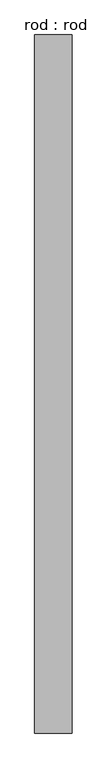
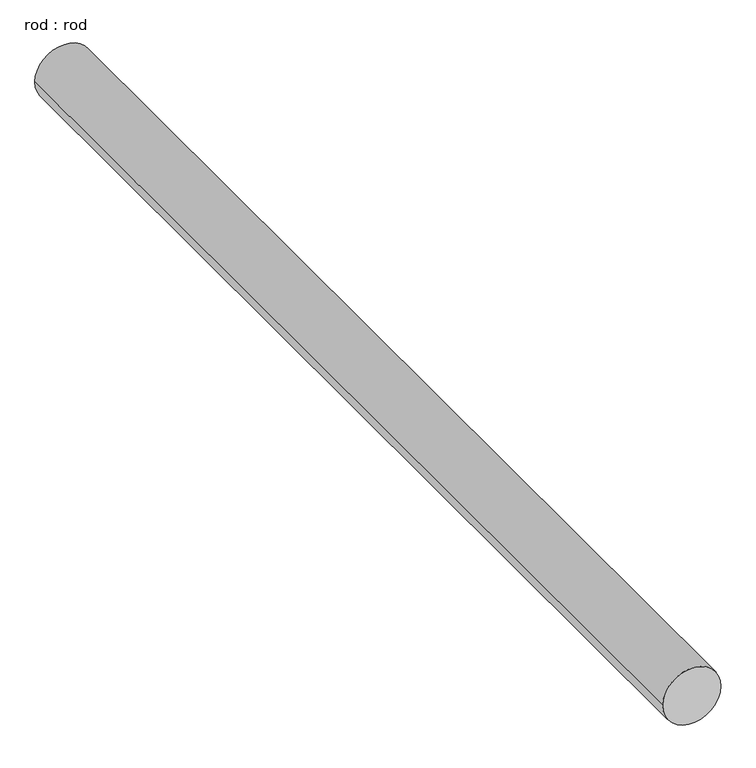
"""IFC4 building model written with IfcOpenShell, lengths in millimetres: proxy geometry, rod : rod."""

import ifcopenshell
import ifcopenshell.guid

model = None  # the IFC model being written
_history = None  # IfcOwnerHistory: only IFC2X3 demands one
_inside = {}  # id of a spatial element -> (the spatial element, [elements in it])
_under = {}  # id of a project, library or spatial element -> (it, [spatial elements below it])
_declared = {}  # id of a project -> (the project, [libraries it declares])
_typed = {}  # id of a type object -> (the type object, [elements of that type])
_made_of = {}  # id of a material, layer set ... -> (it, [elements and type objects made of it])


def new_model(schema):
    """Start an empty IFC model of exactly this schema.

    Asked for "IFC4X3", IfcOpenShell would pick the latest addendum, in which some entities
    have other attributes; the version numbers below select the first issue.
    IFC2X3 requires an IfcOwnerHistory on every rooted entity: one is made here for all.
    """
    global model, _history
    if schema == "IFC4X3":
        model = ifcopenshell.file(schema_version=(4, 3, 0, 0))
    else:
        model = ifcopenshell.file(schema=schema)
    _inside.clear()
    _under.clear()
    _declared.clear()
    _typed.clear()
    _made_of.clear()
    _history = None
    if model.schema == "IFC2X3":
        org = make("IfcOrganization", Name="unknown")
        user = make(
            "IfcPersonAndOrganization",
            ThePerson=make("IfcPerson", FamilyName="unknown"),
            TheOrganization=org,
        )
        app = make(
            "IfcApplication",
            ApplicationDeveloper=org,
            Version="unknown",
            ApplicationFullName="unknown",
            ApplicationIdentifier="unknown",
        )
        _history = make(
            "IfcOwnerHistory",
            OwningUser=user,
            OwningApplication=app,
            ChangeAction="ADDED",
            CreationDate=0,
        )
    return model


def make(cls, **values):
    """One entity of the class cls with the attributes given. An attribute that is None is left unset."""
    return model.create_entity(
        cls, **{name: value for name, value in values.items() if value is not None}
    )


def rooted(cls, **values):
    """An entity with a GlobalId (a new one), such as an element, a storey or a relation."""
    return make(cls, GlobalId=ifcopenshell.guid.new(), OwnerHistory=_history, **values)


def si_unit(unit_type, name, prefix=None):
    """IfcSIUnit, for example si_unit("LENGTHUNIT", "METRE", prefix="MILLI")."""
    return make("IfcSIUnit", UnitType=unit_type, Prefix=prefix, Name=name)


def assignment(units):
    """IfcUnitAssignment: the units of a project."""
    return None if units is None else make("IfcUnitAssignment", Units=units)


def point(xyz):
    """IfcCartesianPoint."""
    return None if xyz is None else make("IfcCartesianPoint", Coordinates=xyz)


def direction(xyz):
    """IfcDirection."""
    return None if xyz is None else make("IfcDirection", DirectionRatios=xyz)


def frame(location, z_axis=None, x_axis=None):
    """IfcAxis2Placement3D, a coordinate frame: its origin and axes. An axis left out is left unset."""
    return make(
        "IfcAxis2Placement3D",
        Location=point(location),
        Axis=direction(z_axis),
        RefDirection=direction(x_axis),
    )


def frame_2d(location, x_axis=None):
    """IfcAxis2Placement2D, a coordinate frame in the plane: its origin and x axis."""
    return make(
        "IfcAxis2Placement2D", Location=point(location), RefDirection=direction(x_axis)
    )


def origin():
    """The frame at (0, 0, 0) with its axes left unset."""
    return frame((0.0, 0.0, 0.0))


def place(relative_to, where):
    """IfcLocalPlacement: puts the frame where relative to a parent placement (None: the world)."""
    return make(
        "IfcLocalPlacement", PlacementRelTo=relative_to, RelativePlacement=where
    )


def context(
    kind, dimensions, precision=None, world=None, true_north=None, identifier=None
):
    """IfcGeometricRepresentationContext, for example the 3D "Model" context."""
    return make(
        "IfcGeometricRepresentationContext",
        ContextIdentifier=identifier,
        ContextType=kind,
        CoordinateSpaceDimension=dimensions,
        Precision=precision,
        WorldCoordinateSystem=world,
        TrueNorth=true_north,
    )


def project(units=None, contexts=None):
    """IfcProject with its units and contexts."""
    return rooted(
        "IfcProject",
        Name="project",
        RepresentationContexts=contexts,
        UnitsInContext=assignment(units),
    )


def spatial(cls, under=None, at=None, **own):
    """A site, building, storey or space (cls), placed at a placement, below another one or the project."""
    s = rooted(cls, ObjectPlacement=at, **own)
    if under is not None:
        _under.setdefault(under.id(), (under, []))[1].append(s)
    return s


def circle_curve(where, radius):
    """IfcCircle in the frame where."""
    return make("IfcCircle", Position=where, Radius=radius)


def trimmed(basis, trim1, trim2, sense, master):
    """IfcTrimmedCurve: the piece of a basis curve between two trims."""
    return make(
        "IfcTrimmedCurve",
        BasisCurve=basis,
        Trim1=trim1,
        Trim2=trim2,
        SenseAgreement=sense,
        MasterRepresentation=master,
    )


def segment(curve, same_sense, transition):
    """IfcCompositeCurveSegment."""
    return make(
        "IfcCompositeCurveSegment",
        Transition=transition,
        SameSense=same_sense,
        ParentCurve=curve,
    )


def composite_curve(segments, self_intersect=None):
    """IfcCompositeCurve: segments joined end to end."""
    return make("IfcCompositeCurve", Segments=segments, SelfIntersect=self_intersect)


def outline(outer, holes=None, kind="AREA"):
    """IfcArbitraryClosedProfileDef: a profile drawn as a closed curve; with holes, ...WithVoids."""
    if holes is None:
        return make("IfcArbitraryClosedProfileDef", ProfileType=kind, OuterCurve=outer)
    return make(
        "IfcArbitraryProfileDefWithVoids",
        ProfileType=kind,
        OuterCurve=outer,
        InnerCurves=holes,
    )


def extrude(swept, where, along, depth):
    """IfcExtrudedAreaSolid: the profile swept, set in the frame where, extruded along a direction by depth."""
    return make(
        "IfcExtrudedAreaSolid",
        SweptArea=swept,
        Position=where,
        ExtrudedDirection=direction(along),
        Depth=depth,
    )


def shape(context_of_items, identifier, shape_type, items):
    """IfcShapeRepresentation: the items that make up one representation, for example the "Body"."""
    return make(
        "IfcShapeRepresentation",
        ContextOfItems=context_of_items,
        RepresentationIdentifier=identifier,
        RepresentationType=shape_type,
        Items=items,
    )


def source(mapping_origin, context_of_items, identifier, shape_type, items):
    """IfcRepresentationMap: a shape defined once, which mapped items show again and again."""
    return make(
        "IfcRepresentationMap",
        MappingOrigin=mapping_origin,
        MappedRepresentation=shape(context_of_items, identifier, shape_type, items),
    )


def transform(
    local_origin,
    x_axis=None,
    y_axis=None,
    z_axis=None,
    scale=None,
    scale2=None,
    scale3=None,
    uniform=True,
):
    """IfcCartesianTransformationOperator3D, or its non-uniform kind. x_axis, y_axis, z_axis: its Axis1, 2, 3."""
    if uniform:
        return make(
            "IfcCartesianTransformationOperator3D",
            Axis1=direction(x_axis),
            Axis2=direction(y_axis),
            LocalOrigin=point(local_origin),
            Scale=scale,
            Axis3=direction(z_axis),
        )
    return make(
        "IfcCartesianTransformationOperator3DnonUniform",
        Axis1=direction(x_axis),
        Axis2=direction(y_axis),
        LocalOrigin=point(local_origin),
        Scale=scale,
        Axis3=direction(z_axis),
        Scale2=scale2,
        Scale3=scale3,
    )


def mapped(mapping_source, mapping_target):
    """IfcMappedItem: shows the shape of a source again, moved by a transform."""
    return make(
        "IfcMappedItem", MappingSource=mapping_source, MappingTarget=mapping_target
    )


def made_of(thing, what):
    """Note that an element or type object is made of a material, layer set ...; save() writes the relation."""
    if what is not None:
        _made_of.setdefault(what.id(), (what, []))[1].append(thing)
    return thing


def element(
    cls,
    number,
    at=None,
    inside=None,
    cuts=None,
    type_object=None,
    material=None,
    context=None,
    identifier="Body",
    shape_type=None,
    held_by="IfcProductDefinitionShape",
    body=None,
    shapes=None,
    **own,
):
    """One element of the class cls, such as IfcWall. Its Tag is "e" and its number.

    at: its placement. inside: the storey or other place that contains it. cuts: it is an
    opening in that element (IfcRelVoidsElement). A single representation is given by context,
    identifier, shape_type and body (its items); several are given by shapes. held_by: the class
    of the entity that holds the representations. save() writes the other relations.
    """
    e = rooted(cls, Tag="e%d" % number, ObjectPlacement=at, **own)
    if body is not None:
        shapes = [shape(context, identifier, shape_type, body)]
    if shapes is not None:
        e.Representation = make(held_by, Representations=shapes)
    if inside is not None:
        _inside.setdefault(inside.id(), (inside, []))[1].append(e)
    if cuts is not None:
        rooted(
            "IfcRelVoidsElement", RelatingBuildingElement=cuts, RelatedOpeningElement=e
        )
    if type_object is not None:
        _typed.setdefault(type_object.id(), (type_object, []))[1].append(e)
    return made_of(e, material)


def aggregate(whole, parts):
    """IfcRelAggregates: a whole, such as a stair, and the parts it consists of."""
    return rooted("IfcRelAggregates", RelatingObject=whole, RelatedObjects=parts)


def save(model, path):
    """Write the relations noted so far, then the file.

    IfcRelAggregates (storeys below a building ...), IfcRelContainedInSpatialStructure (elements
    in a storey), IfcRelDefinesByType, IfcRelAssociatesMaterial and IfcRelDeclares: one each for
    every whole, place, type object, material and project.
    """
    for whole, parts in _under.values():
        aggregate(whole, parts)
    for where, things in _inside.values():
        rooted(
            "IfcRelContainedInSpatialStructure",
            RelatedElements=things,
            RelatingStructure=where,
        )
    for kind, things in _typed.values():
        rooted("IfcRelDefinesByType", RelatedObjects=things, RelatingType=kind)
    for what, things in _made_of.values():
        rooted("IfcRelAssociatesMaterial", RelatedObjects=things, RelatingMaterial=what)
    for by, libraries in _declared.values():
        rooted("IfcRelDeclares", RelatingContext=by, RelatedDefinitions=libraries)
    model.write(path)


def rod_rod_a1119e6b(model_context):
    return source(origin(), model_context, "Body", "SweptSolid", [
        extrude(outline(composite_curve([segment(trimmed(circle_curve(frame_2d((0.0108462, 0.0)), 200.0), [point((0.0108462, 200.0))], [point((0.0108462, -200.0))], False, "CARTESIAN"), True, "CONTINUOUS"), segment(trimmed(circle_curve(frame_2d((0.0108462, 0.0)), 200.0), [point((0.0108462, -200.0))], [point((0.0108462, 200.0))], False, "CARTESIAN"), True, "CONTINUOUS")], self_intersect=False)), frame((0.0, 374.141434, 0.0), z_axis=(0.0, 1.0, 0.0), x_axis=(0.0, 0.0, 1.0)), (0.0, 0.0, 1.0), 7437.1743626),
    ])


if __name__ == "__main__":
    model = new_model("IFC4")
    model_context = context("Model", 3, world=origin())
    ifc_project = project(units=[si_unit("LENGTHUNIT", "METRE", prefix="MILLI")], contexts=[model_context])
    site = spatial("IfcSite", under=ifc_project)
    building = spatial("IfcBuilding", under=site)
    placement = place(None, origin())
    rod_rod_shape = rod_rod_a1119e6b(model_context)
    element("IfcBuildingElementProxy", 1, Name="rod : rod", ObjectType="rod : rod", at=placement, inside=building, context=model_context, shape_type="MappedRepresentation", body=[
        mapped(rod_rod_shape, transform((0.0, 0.0, 0.0), x_axis=(1.0, 0.0, 0.0), y_axis=(0.0, 1.0, 0.0), z_axis=(0.0, 0.0, 1.0))),
    ])
    save(model, "model.ifc")

# Revit data of these elements
# Type "rod : rod"
#   Default Elevation = 0
